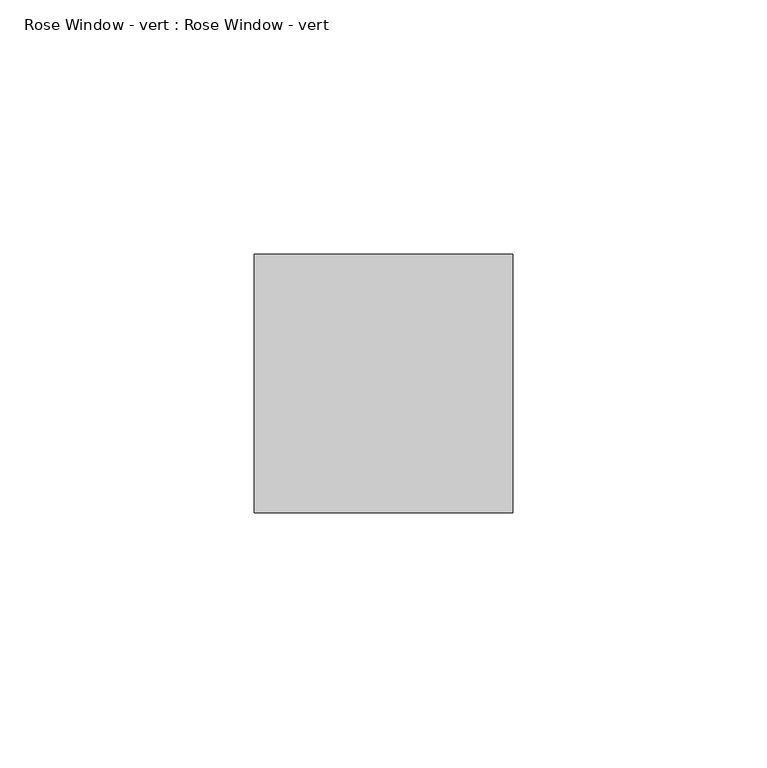
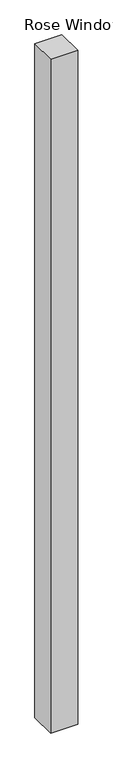
"""IFC4 building model written with IfcOpenShell, lengths in millimetres: furniture geometry, Rose Window - vert : Rose Window - vert."""

from ifc_helpers import new_model, si_unit, frame, origin, place, context, project, spatial, polyline, outline, extrude, source, transform, mapped, element, save


def rose_window_vert_rose_window_vert_7aa00bb0(model_context):
    return source(origin(), model_context, "Body", "SweptSolid", [
        extrude(outline(polyline([(2311.2752098, 15800.565427), (2311.2752098, 15749.765427), (2260.4752098, 15749.765427), (2260.4752098, 15800.565427), (2285.8752098, 15800.565427), (2311.2752098, 15800.565427)])), frame((0.0, 0.0, 3854.45), z_axis=(0.0, 0.0, 1.0), x_axis=(1.0, 0.0, 0.0)), (0.0, 0.0, 1.0), 1336.3742171),
    ])


if __name__ == "__main__":
    model = new_model("IFC4")
    model_context = context("Model", 3, world=origin())
    ifc_project = project(units=[si_unit("LENGTHUNIT", "METRE", prefix="MILLI")], contexts=[model_context])
    site = spatial("IfcSite", under=ifc_project)
    building = spatial("IfcBuilding", under=site)
    placement = place(None, origin())
    rose_window_vert_rose_window_vert_shape = rose_window_vert_rose_window_vert_7aa00bb0(model_context)
    element("IfcFurniture", 1, ObjectType="Rose Window - vert : Rose Window - vert", at=placement, inside=building, context=model_context, shape_type="MappedRepresentation", body=[
        mapped(rose_window_vert_rose_window_vert_shape, transform((0.0, 0.0, 0.0), x_axis=(1.0, 0.0, 0.0), y_axis=(0.0, 1.0, 0.0), z_axis=(0.0, 0.0, 1.0))),
    ])
    save(model, "model.ifc")

# Revit data of these elements
# Type "Rose Window - vert : Rose Window - vert"
#   COBie.Type = no
# Element 1 (IfcFurniture, "Rose Window - vert : Rose Window - vert")
#   Materials on its faces: "Trim - White"
# Materials
#   "Trim - White": class "Wood", colour RGB 255 255 255, transparency 0, Cost = 0
